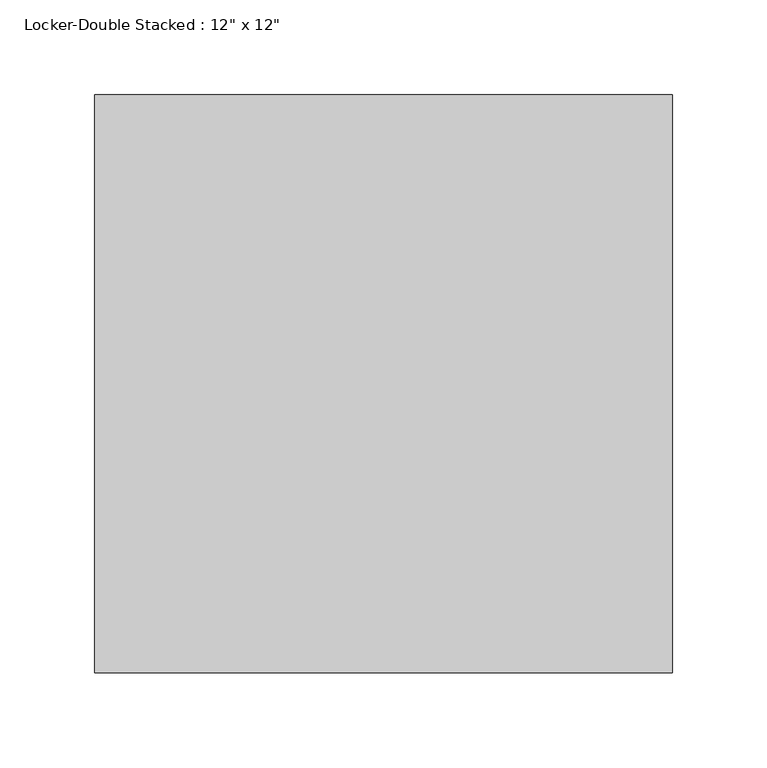
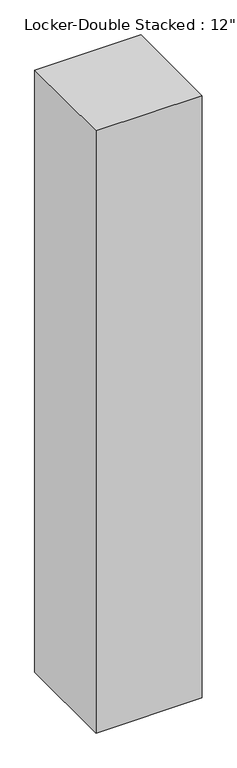
"""IFC4 building model written with IfcOpenShell, lengths in millimetres: furniture geometry."""

from ifc_helpers import new_model, si_unit, origin, place, context, project, spatial, faceted_brep, source, transform, mapped, element, save


def furniture_8e8d9ebb(model_context):
    return source(origin(), model_context, "Body", "Brep", [
        faceted_brep([(152.4, 152.4, 1828.8), (-152.4, 152.4, 1828.8), (-152.4, -152.4, 1828.8), (152.4, -152.4, 1828.8), (152.4, 152.4, 0.0), (152.4, -152.4, 0.0), (-152.4, -152.4, 0.0), (-152.4, 152.4, 0.0), (127.0, 152.4, 889.0), (-127.0, 152.4, 889.0), (-127.0, 152.4, 76.2), (127.0, 152.4, 76.2), (-127.0, 152.4, 1752.6), (-127.0, 152.4, 939.8), (127.0, 152.4, 939.8), (127.0, 152.4, 1752.6), (127.0, 146.05, 76.2), (-127.0, 146.05, 76.2), (-127.0, 146.05, 889.0), (127.0, 146.05, 889.0), (127.0, 146.05, 1752.6), (127.0, 146.05, 939.8), (-127.0, 146.05, 939.8), (-127.0, 146.05, 1752.6)], [[[0, 1, 2, 3]], [[4, 5, 6, 7]], [[3, 5, 4, 0]], [[2, 6, 5, 3]], [[1, 7, 6, 2]], [[0, 4, 7, 1], [8, 9, 10, 11], [12, 13, 14, 15]], [[16, 17, 18, 19]], [[19, 8, 11, 16]], [[18, 9, 8, 19]], [[17, 10, 9, 18]], [[16, 11, 10, 17]], [[20, 21, 22, 23]], [[23, 12, 15, 20]], [[22, 13, 12, 23]], [[21, 14, 13, 22]], [[20, 15, 14, 21]]]),
    ])


if __name__ == "__main__":
    model = new_model("IFC4")
    model_context = context("Model", 3, world=origin())
    ifc_project = project(units=[si_unit("LENGTHUNIT", "METRE", prefix="MILLI")], contexts=[model_context])
    site = spatial("IfcSite", under=ifc_project)
    building = spatial("IfcBuilding", under=site)
    placement = place(None, origin())
    furniture_shape = furniture_8e8d9ebb(model_context)
    element("IfcFurniture", 1, ObjectType="Locker-Double Stacked : 12\" x 12\"", at=placement, inside=building, context=model_context, shape_type="MappedRepresentation", body=[
        mapped(furniture_shape, transform((0.0, 0.0, 0.0), x_axis=(1.0, 0.0, 0.0), y_axis=(0.0, 1.0, 0.0), z_axis=(0.0, 0.0, 1.0))),
    ])
    save(model, "model.ifc")

# Revit data of these elements
# Type "Locker-Double Stacked : 12\" x 12\""
#   Assembly Code = "E2010"
#   Depth = 1' - 0"
#   Height = 6' - 0"
#   Width = 1' - 0"
#   Material = Metal - Paint Finish - Dark Gray, Matte
# Element 1 (IfcFurniture, "Locker-Double Stacked : 12\" x 12\"")
#   Materials on its faces: "Metal - Paint Finish - Dark Gray, Matte"
# Materials
#   "Metal - Paint Finish - Dark Gray, Matte": class "Metal", colour RGB 98 98 98, transparency 0
